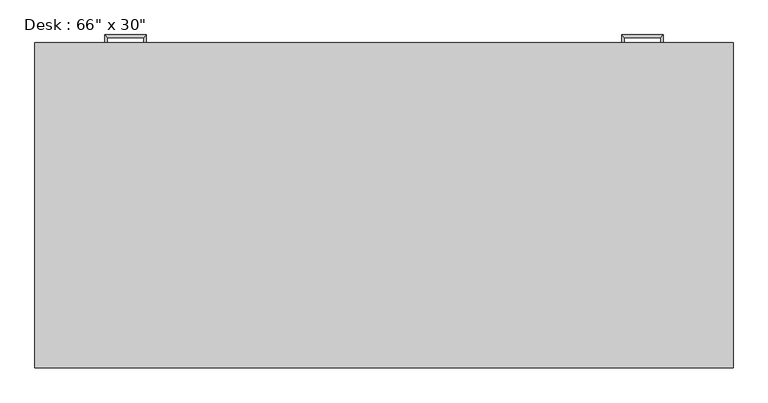
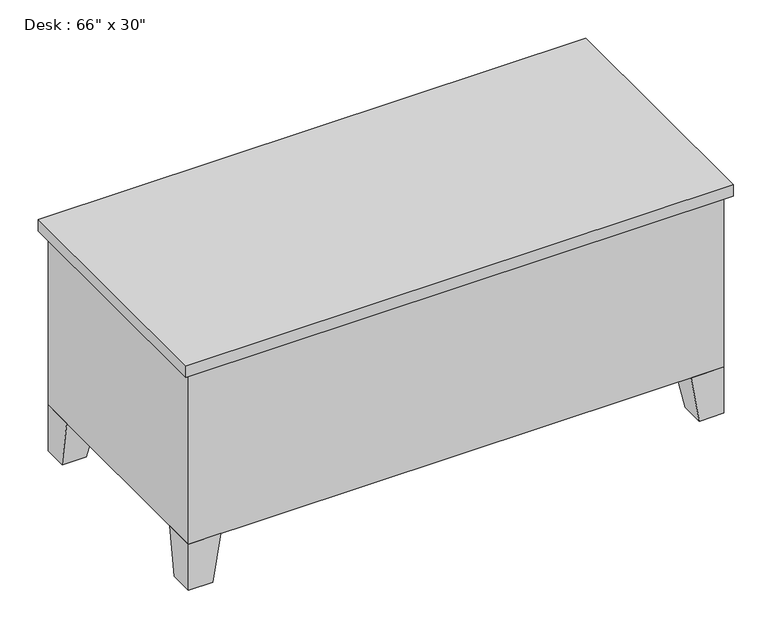
"""IFC4 building model written with IfcOpenShell, lengths in millimetres: furniture geometry."""

import ifcopenshell
import ifcopenshell.guid

model = None  # the IFC model being written
_history = None  # IfcOwnerHistory: only IFC2X3 demands one
_inside = {}  # id of a spatial element -> (the spatial element, [elements in it])
_under = {}  # id of a project, library or spatial element -> (it, [spatial elements below it])
_declared = {}  # id of a project -> (the project, [libraries it declares])
_typed = {}  # id of a type object -> (the type object, [elements of that type])
_made_of = {}  # id of a material, layer set ... -> (it, [elements and type objects made of it])


def new_model(schema):
    """Start an empty IFC model of exactly this schema.

    Asked for "IFC4X3", IfcOpenShell would pick the latest addendum, in which some entities
    have other attributes; the version numbers below select the first issue.
    IFC2X3 requires an IfcOwnerHistory on every rooted entity: one is made here for all.
    """
    global model, _history
    if schema == "IFC4X3":
        model = ifcopenshell.file(schema_version=(4, 3, 0, 0))
    else:
        model = ifcopenshell.file(schema=schema)
    _inside.clear()
    _under.clear()
    _declared.clear()
    _typed.clear()
    _made_of.clear()
    _history = None
    if model.schema == "IFC2X3":
        org = make("IfcOrganization", Name="unknown")
        user = make(
            "IfcPersonAndOrganization",
            ThePerson=make("IfcPerson", FamilyName="unknown"),
            TheOrganization=org,
        )
        app = make(
            "IfcApplication",
            ApplicationDeveloper=org,
            Version="unknown",
            ApplicationFullName="unknown",
            ApplicationIdentifier="unknown",
        )
        _history = make(
            "IfcOwnerHistory",
            OwningUser=user,
            OwningApplication=app,
            ChangeAction="ADDED",
            CreationDate=0,
        )
    return model


def make(cls, **values):
    """One entity of the class cls with the attributes given. An attribute that is None is left unset."""
    return model.create_entity(
        cls, **{name: value for name, value in values.items() if value is not None}
    )


def rooted(cls, **values):
    """An entity with a GlobalId (a new one), such as an element, a storey or a relation."""
    return make(cls, GlobalId=ifcopenshell.guid.new(), OwnerHistory=_history, **values)


def si_unit(unit_type, name, prefix=None):
    """IfcSIUnit, for example si_unit("LENGTHUNIT", "METRE", prefix="MILLI")."""
    return make("IfcSIUnit", UnitType=unit_type, Prefix=prefix, Name=name)


def assignment(units):
    """IfcUnitAssignment: the units of a project."""
    return None if units is None else make("IfcUnitAssignment", Units=units)


def point(xyz):
    """IfcCartesianPoint."""
    return None if xyz is None else make("IfcCartesianPoint", Coordinates=xyz)


def direction(xyz):
    """IfcDirection."""
    return None if xyz is None else make("IfcDirection", DirectionRatios=xyz)


def frame(location, z_axis=None, x_axis=None):
    """IfcAxis2Placement3D, a coordinate frame: its origin and axes. An axis left out is left unset."""
    return make(
        "IfcAxis2Placement3D",
        Location=point(location),
        Axis=direction(z_axis),
        RefDirection=direction(x_axis),
    )


def origin():
    """The frame at (0, 0, 0) with its axes left unset."""
    return frame((0.0, 0.0, 0.0))


def place(relative_to, where):
    """IfcLocalPlacement: puts the frame where relative to a parent placement (None: the world)."""
    return make(
        "IfcLocalPlacement", PlacementRelTo=relative_to, RelativePlacement=where
    )


def context(
    kind, dimensions, precision=None, world=None, true_north=None, identifier=None
):
    """IfcGeometricRepresentationContext, for example the 3D "Model" context."""
    return make(
        "IfcGeometricRepresentationContext",
        ContextIdentifier=identifier,
        ContextType=kind,
        CoordinateSpaceDimension=dimensions,
        Precision=precision,
        WorldCoordinateSystem=world,
        TrueNorth=true_north,
    )


def project(units=None, contexts=None):
    """IfcProject with its units and contexts."""
    return rooted(
        "IfcProject",
        Name="project",
        RepresentationContexts=contexts,
        UnitsInContext=assignment(units),
    )


def spatial(cls, under=None, at=None, **own):
    """A site, building, storey or space (cls), placed at a placement, below another one or the project."""
    s = rooted(cls, ObjectPlacement=at, **own)
    if under is not None:
        _under.setdefault(under.id(), (under, []))[1].append(s)
    return s


def polyline(points):
    """IfcPolyline through the points."""
    return make("IfcPolyline", Points=[point(p) for p in points])


def outline(outer, holes=None, kind="AREA"):
    """IfcArbitraryClosedProfileDef: a profile drawn as a closed curve; with holes, ...WithVoids."""
    if holes is None:
        return make("IfcArbitraryClosedProfileDef", ProfileType=kind, OuterCurve=outer)
    return make(
        "IfcArbitraryProfileDefWithVoids",
        ProfileType=kind,
        OuterCurve=outer,
        InnerCurves=holes,
    )


def extrude(swept, where, along, depth):
    """IfcExtrudedAreaSolid: the profile swept, set in the frame where, extruded along a direction by depth."""
    return make(
        "IfcExtrudedAreaSolid",
        SweptArea=swept,
        Position=where,
        ExtrudedDirection=direction(along),
        Depth=depth,
    )


def faces_of(points, faces, orient=None, outer=None):
    """IfcFace entities. A face is a list of loops; a loop is a list of indices into points, from 0.

    orient and outer hold one flag for each loop. By default every Orientation is true, the
    first loop of a face is its IfcFaceOuterBound and the others are IfcFaceBound.
    """
    made = []
    for i, loops in enumerate(faces):
        bounds = []
        for j, loop in enumerate(loops):
            is_outer = j == 0 if outer is None else outer[i][j]
            bounds.append(
                make(
                    "IfcFaceOuterBound" if is_outer else "IfcFaceBound",
                    Bound=make("IfcPolyLoop", Polygon=[points[k] for k in loop]),
                    Orientation=True if orient is None else orient[i][j],
                )
            )
        made.append(make("IfcFace", Bounds=bounds))
    return made


def faceted_brep(points, faces, orient=None, outer=None, voids=None):
    """IfcFacetedBrep: a solid bounded by flat faces; with voids (closed shells), ...WithVoids."""
    shared = [point(p) for p in points]
    hull = make("IfcClosedShell", CfsFaces=faces_of(shared, faces, orient, outer))
    if voids is None:
        return make("IfcFacetedBrep", Outer=hull)
    return make(
        "IfcFacetedBrepWithVoids",
        Outer=hull,
        Voids=[
            make(cls, CfsFaces=faces_of(shared, fs, o, b)) for cls, fs, o, b in voids
        ],
    )


def shape(context_of_items, identifier, shape_type, items):
    """IfcShapeRepresentation: the items that make up one representation, for example the "Body"."""
    return make(
        "IfcShapeRepresentation",
        ContextOfItems=context_of_items,
        RepresentationIdentifier=identifier,
        RepresentationType=shape_type,
        Items=items,
    )


def source(mapping_origin, context_of_items, identifier, shape_type, items):
    """IfcRepresentationMap: a shape defined once, which mapped items show again and again."""
    return make(
        "IfcRepresentationMap",
        MappingOrigin=mapping_origin,
        MappedRepresentation=shape(context_of_items, identifier, shape_type, items),
    )


def transform(
    local_origin,
    x_axis=None,
    y_axis=None,
    z_axis=None,
    scale=None,
    scale2=None,
    scale3=None,
    uniform=True,
):
    """IfcCartesianTransformationOperator3D, or its non-uniform kind. x_axis, y_axis, z_axis: its Axis1, 2, 3."""
    if uniform:
        return make(
            "IfcCartesianTransformationOperator3D",
            Axis1=direction(x_axis),
            Axis2=direction(y_axis),
            LocalOrigin=point(local_origin),
            Scale=scale,
            Axis3=direction(z_axis),
        )
    return make(
        "IfcCartesianTransformationOperator3DnonUniform",
        Axis1=direction(x_axis),
        Axis2=direction(y_axis),
        LocalOrigin=point(local_origin),
        Scale=scale,
        Axis3=direction(z_axis),
        Scale2=scale2,
        Scale3=scale3,
    )


def mapped(mapping_source, mapping_target):
    """IfcMappedItem: shows the shape of a source again, moved by a transform."""
    return make(
        "IfcMappedItem", MappingSource=mapping_source, MappingTarget=mapping_target
    )


def made_of(thing, what):
    """Note that an element or type object is made of a material, layer set ...; save() writes the relation."""
    if what is not None:
        _made_of.setdefault(what.id(), (what, []))[1].append(thing)
    return thing


def element(
    cls,
    number,
    at=None,
    inside=None,
    cuts=None,
    type_object=None,
    material=None,
    context=None,
    identifier="Body",
    shape_type=None,
    held_by="IfcProductDefinitionShape",
    body=None,
    shapes=None,
    **own,
):
    """One element of the class cls, such as IfcWall. Its Tag is "e" and its number.

    at: its placement. inside: the storey or other place that contains it. cuts: it is an
    opening in that element (IfcRelVoidsElement). A single representation is given by context,
    identifier, shape_type and body (its items); several are given by shapes. held_by: the class
    of the entity that holds the representations. save() writes the other relations.
    """
    e = rooted(cls, Tag="e%d" % number, ObjectPlacement=at, **own)
    if body is not None:
        shapes = [shape(context, identifier, shape_type, body)]
    if shapes is not None:
        e.Representation = make(held_by, Representations=shapes)
    if inside is not None:
        _inside.setdefault(inside.id(), (inside, []))[1].append(e)
    if cuts is not None:
        rooted(
            "IfcRelVoidsElement", RelatingBuildingElement=cuts, RelatedOpeningElement=e
        )
    if type_object is not None:
        _typed.setdefault(type_object.id(), (type_object, []))[1].append(e)
    return made_of(e, material)


def aggregate(whole, parts):
    """IfcRelAggregates: a whole, such as a stair, and the parts it consists of."""
    return rooted("IfcRelAggregates", RelatingObject=whole, RelatedObjects=parts)


def save(model, path):
    """Write the relations noted so far, then the file.

    IfcRelAggregates (storeys below a building ...), IfcRelContainedInSpatialStructure (elements
    in a storey), IfcRelDefinesByType, IfcRelAssociatesMaterial and IfcRelDeclares: one each for
    every whole, place, type object, material and project.
    """
    for whole, parts in _under.values():
        aggregate(whole, parts)
    for where, things in _inside.values():
        rooted(
            "IfcRelContainedInSpatialStructure",
            RelatedElements=things,
            RelatingStructure=where,
        )
    for kind, things in _typed.values():
        rooted("IfcRelDefinesByType", RelatedObjects=things, RelatingType=kind)
    for what, things in _made_of.values():
        rooted("IfcRelAssociatesMaterial", RelatedObjects=things, RelatingMaterial=what)
    for by, libraries in _declared.values():
        rooted("IfcRelDeclares", RelatingContext=by, RelatedDefinitions=libraries)
    model.write(path)


def furniture_bcdaa455(model_context):
    return source(origin(), model_context, "Body", "SolidModel", [
        extrude(outline(polyline([(1657.35, 762.0), (1289.05, 762.0), (1289.05, 774.7), (1657.35, 774.7), (1657.35, 762.0)])), frame((0.0, 0.0, 603.25), z_axis=(0.0, 0.0, 1.0), x_axis=(1.0, 0.0, 0.0)), (0.0, 0.0, 1.0), 101.6),
        extrude(outline(polyline([(1657.35, 762.0), (1289.05, 762.0), (1289.05, 774.7), (1657.35, 774.7), (1657.35, 762.0)])), frame((0.0, 0.0, 171.45), z_axis=(0.0, 0.0, 1.0), x_axis=(1.0, 0.0, 0.0)), (0.0, 0.0, 1.0), 412.75),
        extrude(outline(polyline([(387.35, 762.0), (19.05, 762.0), (19.05, 774.7), (387.35, 774.7), (387.35, 762.0)])), frame((0.0, 0.0, 603.25), z_axis=(0.0, 0.0, 1.0), x_axis=(1.0, 0.0, 0.0)), (0.0, 0.0, 1.0), 101.6),
        extrude(outline(polyline([(387.35, 762.0), (19.05, 762.0), (19.05, 774.7), (387.35, 774.7), (387.35, 762.0)])), frame((0.0, 0.0, 171.45), z_axis=(0.0, 0.0, 1.0), x_axis=(1.0, 0.0, 0.0)), (0.0, 0.0, 1.0), 171.45),
        extrude(outline(polyline([(387.35, 762.0), (19.05, 762.0), (19.05, 774.7), (387.35, 774.7), (387.35, 762.0)])), frame((0.0, 0.0, 482.6), z_axis=(0.0, 0.0, 1.0), x_axis=(1.0, 0.0, 0.0)), (0.0, 0.0, 1.0), 101.6),
        extrude(outline(polyline([(387.35, 762.0), (19.05, 762.0), (19.05, 774.7), (387.35, 774.7), (387.35, 762.0)])), frame((0.0, 0.0, 361.95), z_axis=(0.0, 0.0, 1.0), x_axis=(1.0, 0.0, 0.0)), (0.0, 0.0, 1.0), 101.6),
        faceted_brep([(1574.8, 762.0, 152.4), (1574.8, 660.4, 152.4), (1676.4, 660.4, 152.4), (1676.4, 762.0, 152.4), (1600.2, 762.0, 0.0), (1676.4, 762.0, 0.0), (1676.4, 685.8, 0.0), (1600.2, 685.8, 0.0)], [[[0, 1, 2, 3]], [[4, 5, 6, 7]], [[4, 7, 1, 0]], [[7, 6, 2, 1]], [[6, 5, 3, 2]], [[5, 4, 0, 3]]]),
        faceted_brep([(1574.8, 0.0, 152.4), (1676.4, 0.0, 152.4), (1676.4, 101.6, 152.4), (1574.8, 101.6, 152.4), (1600.2, 0.0, 0.0), (1600.2, 76.2, 0.0), (1676.4, 76.2, 0.0), (1676.4, 0.0, 0.0)], [[[0, 1, 2, 3]], [[4, 5, 6, 7]], [[4, 7, 1, 0]], [[7, 6, 2, 1]], [[6, 5, 3, 2]], [[5, 4, 0, 3]]]),
        faceted_brep([(101.6, 0.0, 152.4), (101.6, 101.6, 152.4), (0.0, 101.6, 152.4), (0.0, 0.0, 152.4), (76.2, 0.0, 0.0), (0.0, 0.0, 0.0), (0.0, 76.2, 0.0), (76.2, 76.2, 0.0)], [[[0, 1, 2, 3]], [[4, 5, 6, 7]], [[4, 7, 1, 0]], [[7, 6, 2, 1]], [[6, 5, 3, 2]], [[5, 4, 0, 3]]]),
        faceted_brep([(101.6, 762.0, 152.4), (0.0, 762.0, 152.4), (0.0, 660.4, 152.4), (101.6, 660.4, 152.4), (76.2, 762.0, 0.0), (76.2, 685.8, 0.0), (0.0, 685.8, 0.0), (0.0, 762.0, 0.0)], [[[0, 1, 2, 3]], [[4, 5, 6, 7]], [[4, 7, 1, 0]], [[7, 6, 2, 1]], [[6, 5, 3, 2]], [[5, 4, 0, 3]]]),
        extrude(outline(polyline([(1695.45, 781.05), (1695.45, -19.05), (-19.05, -19.05), (-19.05, 781.05), (1695.45, 781.05)])), frame((0.0, 0.0, 723.9), z_axis=(0.0, 0.0, 1.0), x_axis=(1.0, 0.0, 0.0)), (0.0, 0.0, 1.0), 38.1),
        extrude(outline(polyline([(406.4, 762.0), (406.4, 50.8), (1270.0, 50.8), (1270.0, 762.0), (1676.4, 762.0), (1676.4, 0.0), (0.0, 0.0), (0.0, 762.0), (406.4, 762.0)])), frame((0.0, 0.0, 152.4), z_axis=(0.0, 0.0, 1.0), x_axis=(1.0, 0.0, 0.0)), (0.0, 0.0, 1.0), 571.5),
        faceted_brep([(1517.65, 774.7, 546.1), (1517.65, 774.7, 533.4), (1524.0, 774.7, 533.4), (1524.0, 774.7, 546.1), (1517.65, 793.75, 546.1), (1517.65, 793.75, 533.4), (1524.0, 800.1, 533.4), (1524.0, 800.1, 546.1), (1428.75, 793.75, 546.1), (1428.75, 793.75, 533.4), (1422.4, 800.1, 533.4), (1422.4, 800.1, 546.1), (1428.75, 774.7, 546.1), (1422.4, 774.7, 546.1), (1422.4, 774.7, 533.4), (1428.75, 774.7, 533.4)], [[[0, 1, 2, 3]], [[1, 0, 4, 5]], [[2, 1, 5, 6]], [[3, 2, 6, 7]], [[0, 3, 7, 4]], [[5, 4, 8, 9]], [[6, 5, 9, 10]], [[7, 6, 10, 11]], [[4, 7, 11, 8]], [[12, 13, 14, 15]], [[9, 8, 12, 15]], [[10, 9, 15, 14]], [[11, 10, 14, 13]], [[8, 11, 13, 12]]]),
        faceted_brep([(1517.65, 774.7, 666.75), (1517.65, 774.7, 654.05), (1524.0, 774.7, 654.05), (1524.0, 774.7, 666.75), (1517.65, 793.75, 666.75), (1517.65, 793.75, 654.05), (1524.0, 800.1, 654.05), (1524.0, 800.1, 666.75), (1428.75, 793.75, 666.75), (1428.75, 793.75, 654.05), (1422.4, 800.1, 654.05), (1422.4, 800.1, 666.75), (1428.75, 774.7, 666.75), (1422.4, 774.7, 666.75), (1422.4, 774.7, 654.05), (1428.75, 774.7, 654.05)], [[[0, 1, 2, 3]], [[1, 0, 4, 5]], [[2, 1, 5, 6]], [[3, 2, 6, 7]], [[0, 3, 7, 4]], [[5, 4, 8, 9]], [[6, 5, 9, 10]], [[7, 6, 10, 11]], [[4, 7, 11, 8]], [[12, 13, 14, 15]], [[9, 8, 12, 15]], [[10, 9, 15, 14]], [[11, 10, 14, 13]], [[8, 11, 13, 12]]]),
        faceted_brep([(158.75, 774.7, 304.8), (152.4, 774.7, 304.8), (152.4, 774.7, 292.1), (158.75, 774.7, 292.1), (158.75, 793.75, 304.8), (152.4, 800.1, 304.8), (152.4, 800.1, 292.1), (158.75, 793.75, 292.1), (247.65, 793.75, 304.8), (254.0, 800.1, 304.8), (254.0, 800.1, 292.1), (247.65, 793.75, 292.1), (247.65, 774.7, 304.8), (247.65, 774.7, 292.1), (254.0, 774.7, 292.1), (254.0, 774.7, 304.8)], [[[0, 1, 2, 3]], [[1, 0, 4, 5]], [[2, 1, 5, 6]], [[3, 2, 6, 7]], [[0, 3, 7, 4]], [[5, 4, 8, 9]], [[6, 5, 9, 10]], [[7, 6, 10, 11]], [[4, 7, 11, 8]], [[12, 13, 14, 15]], [[9, 8, 12, 15]], [[10, 9, 15, 14]], [[11, 10, 14, 13]], [[8, 11, 13, 12]]]),
        faceted_brep([(158.75, 774.7, 425.45), (152.4, 774.7, 425.45), (152.4, 774.7, 412.75), (158.75, 774.7, 412.75), (158.75, 793.75, 425.45), (152.4, 800.1, 425.45), (152.4, 800.1, 412.75), (158.75, 793.75, 412.75), (247.65, 793.75, 425.45), (254.0, 800.1, 425.45), (254.0, 800.1, 412.75), (247.65, 793.75, 412.75), (247.65, 774.7, 425.45), (247.65, 774.7, 412.75), (254.0, 774.7, 412.75), (254.0, 774.7, 425.45)], [[[0, 1, 2, 3]], [[1, 0, 4, 5]], [[2, 1, 5, 6]], [[3, 2, 6, 7]], [[0, 3, 7, 4]], [[5, 4, 8, 9]], [[6, 5, 9, 10]], [[7, 6, 10, 11]], [[4, 7, 11, 8]], [[12, 13, 14, 15]], [[9, 8, 12, 15]], [[10, 9, 15, 14]], [[11, 10, 14, 13]], [[8, 11, 13, 12]]]),
        faceted_brep([(158.75, 774.7, 546.1), (152.4, 774.7, 546.1), (152.4, 774.7, 533.4), (158.75, 774.7, 533.4), (158.75, 793.75, 546.1), (152.4, 800.1, 546.1), (152.4, 800.1, 533.4), (158.75, 793.75, 533.4), (247.65, 793.75, 546.1), (254.0, 800.1, 546.1), (254.0, 800.1, 533.4), (247.65, 793.75, 533.4), (247.65, 774.7, 546.1), (247.65, 774.7, 533.4), (254.0, 774.7, 533.4), (254.0, 774.7, 546.1)], [[[0, 1, 2, 3]], [[1, 0, 4, 5]], [[2, 1, 5, 6]], [[3, 2, 6, 7]], [[0, 3, 7, 4]], [[5, 4, 8, 9]], [[6, 5, 9, 10]], [[7, 6, 10, 11]], [[4, 7, 11, 8]], [[12, 13, 14, 15]], [[9, 8, 12, 15]], [[10, 9, 15, 14]], [[11, 10, 14, 13]], [[8, 11, 13, 12]]]),
        faceted_brep([(158.75, 774.7, 666.75), (152.4, 774.7, 666.75), (152.4, 774.7, 654.05), (158.75, 774.7, 654.05), (158.75, 793.75, 666.75), (152.4, 800.1, 666.75), (152.4, 800.1, 654.05), (158.75, 793.75, 654.05), (247.65, 793.75, 666.75), (254.0, 800.1, 666.75), (254.0, 800.1, 654.05), (247.65, 793.75, 654.05), (247.65, 774.7, 666.75), (247.65, 774.7, 654.05), (254.0, 774.7, 654.05), (254.0, 774.7, 666.75)], [[[0, 1, 2, 3]], [[1, 0, 4, 5]], [[2, 1, 5, 6]], [[3, 2, 6, 7]], [[0, 3, 7, 4]], [[5, 4, 8, 9]], [[6, 5, 9, 10]], [[7, 6, 10, 11]], [[4, 7, 11, 8]], [[12, 13, 14, 15]], [[9, 8, 12, 15]], [[10, 9, 15, 14]], [[11, 10, 14, 13]], [[8, 11, 13, 12]]]),
    ])


if __name__ == "__main__":
    model = new_model("IFC4")
    model_context = context("Model", 3, world=origin())
    ifc_project = project(units=[si_unit("LENGTHUNIT", "METRE", prefix="MILLI")], contexts=[model_context])
    site = spatial("IfcSite", under=ifc_project)
    building = spatial("IfcBuilding", under=site)
    placement = place(None, origin())
    furniture_shape = furniture_bcdaa455(model_context)
    element("IfcFurniture", 1, ObjectType="Desk : 66\" x 30\"", at=placement, inside=building, context=model_context, shape_type="MappedRepresentation", body=[
        mapped(furniture_shape, transform((0.0, 0.0, 0.0), x_axis=(1.0, 0.0, 0.0), y_axis=(0.0, 1.0, 0.0), z_axis=(0.0, 0.0, 1.0))),
    ])
    save(model, "model.ifc")

# Revit data of these elements
# Type "Desk : 66\" x 30\""
#   Model = "TSK-5679"
#   Manufacturer = "Acme Furniture"
#   Type Mark = "DK-2"
#   Assembly Code = "E2020200"
#   Cost = 1050
#   Depth = 2' - 6"
#   Height = 2' - 6"
#   Leg Height = 0' - 6"
#   Width = 5' - 6"
#   Body Material = Laminate, Ivory, Matte
#   Handle/Leg Material = Steel, Chrome Plated
#   Top Material = Cherry
#   Default Elevation = 0
# Element 1 (IfcFurniture, "Desk : 66\" x 30\"")
#   Materials on its faces: "Steel, Chrome Plated", "Laminate, Ivory, Matte", "Cherry"
# Materials
#   "Laminate, Ivory, Matte": class "Plastic", colour RGB 247 247 239, transparency 0, Description = "Plastic Laminate - Ivory, Matte", Cost = 0
#   "Steel, Chrome Plated": class "Metal", colour RGB 17 17 17, transparency 0, Description = "Chromiuim plated steel", Cost = 0
#   "Cherry": class "Wood", colour RGB 226 177 128, transparency 0, Description = "Prunus Serotina", Cost = 0
